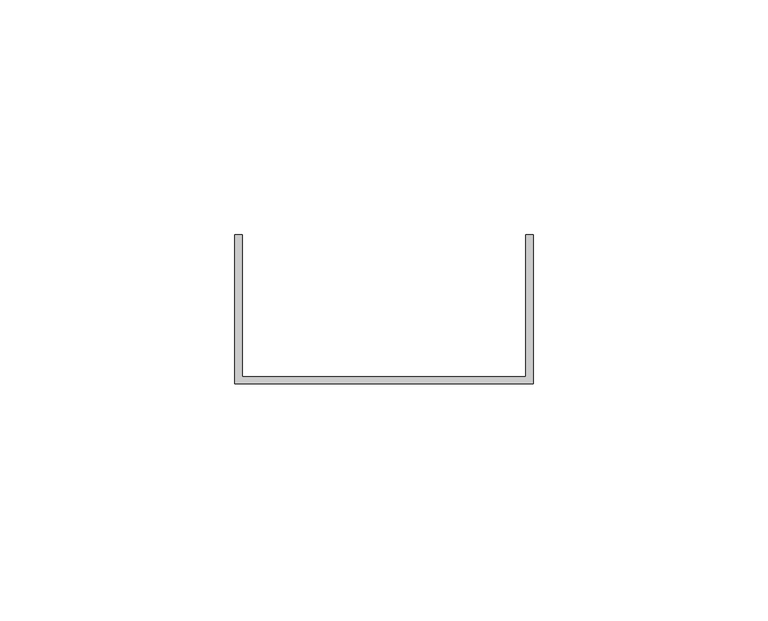
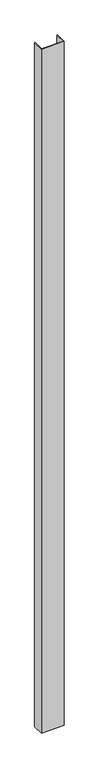
"""IFC4 building model written with IfcOpenShell, lengths in millimetres: proxy geometry, Generic Models 7:Generic Models 1:3:Generic Models 1:3 : Generic Models 7:Generic Models 1:305549:3:Generic Models 1:3:Generic Models 1:3 : Generic Models 7:Generic Models 1:305549:3 : Generic Models 7:Generic Models 1:3:Generic Models 1:3 : Generic Models 7:Generic Models 1:305549:301244:29 : Generic Models 7:Generic Models 1:3:Generic Models 1:3 : Generic Models 7:Generic Models 1:305549:3:Generic Models 1:3:Generic Models 1:3 : Generic Models 7:Generic Models 1:305549:3 : Generic Models 7:Generic Models 1:3:Generic Models 1:3 : Generic Models 7:Generic Models 1:305549:301244:308848."""

import ifcopenshell
import ifcopenshell.guid

model = None  # the IFC model being written
_history = None  # IfcOwnerHistory: only IFC2X3 demands one
_inside = {}  # id of a spatial element -> (the spatial element, [elements in it])
_under = {}  # id of a project, library or spatial element -> (it, [spatial elements below it])
_declared = {}  # id of a project -> (the project, [libraries it declares])
_typed = {}  # id of a type object -> (the type object, [elements of that type])
_made_of = {}  # id of a material, layer set ... -> (it, [elements and type objects made of it])


def new_model(schema):
    """Start an empty IFC model of exactly this schema.

    Asked for "IFC4X3", IfcOpenShell would pick the latest addendum, in which some entities
    have other attributes; the version numbers below select the first issue.
    IFC2X3 requires an IfcOwnerHistory on every rooted entity: one is made here for all.
    """
    global model, _history
    if schema == "IFC4X3":
        model = ifcopenshell.file(schema_version=(4, 3, 0, 0))
    else:
        model = ifcopenshell.file(schema=schema)
    _inside.clear()
    _under.clear()
    _declared.clear()
    _typed.clear()
    _made_of.clear()
    _history = None
    if model.schema == "IFC2X3":
        org = make("IfcOrganization", Name="unknown")
        user = make(
            "IfcPersonAndOrganization",
            ThePerson=make("IfcPerson", FamilyName="unknown"),
            TheOrganization=org,
        )
        app = make(
            "IfcApplication",
            ApplicationDeveloper=org,
            Version="unknown",
            ApplicationFullName="unknown",
            ApplicationIdentifier="unknown",
        )
        _history = make(
            "IfcOwnerHistory",
            OwningUser=user,
            OwningApplication=app,
            ChangeAction="ADDED",
            CreationDate=0,
        )
    return model


def make(cls, **values):
    """One entity of the class cls with the attributes given. An attribute that is None is left unset."""
    return model.create_entity(
        cls, **{name: value for name, value in values.items() if value is not None}
    )


def rooted(cls, **values):
    """An entity with a GlobalId (a new one), such as an element, a storey or a relation."""
    return make(cls, GlobalId=ifcopenshell.guid.new(), OwnerHistory=_history, **values)


def si_unit(unit_type, name, prefix=None):
    """IfcSIUnit, for example si_unit("LENGTHUNIT", "METRE", prefix="MILLI")."""
    return make("IfcSIUnit", UnitType=unit_type, Prefix=prefix, Name=name)


def assignment(units):
    """IfcUnitAssignment: the units of a project."""
    return None if units is None else make("IfcUnitAssignment", Units=units)


def point(xyz):
    """IfcCartesianPoint."""
    return None if xyz is None else make("IfcCartesianPoint", Coordinates=xyz)


def direction(xyz):
    """IfcDirection."""
    return None if xyz is None else make("IfcDirection", DirectionRatios=xyz)


def frame(location, z_axis=None, x_axis=None):
    """IfcAxis2Placement3D, a coordinate frame: its origin and axes. An axis left out is left unset."""
    return make(
        "IfcAxis2Placement3D",
        Location=point(location),
        Axis=direction(z_axis),
        RefDirection=direction(x_axis),
    )


def origin():
    """The frame at (0, 0, 0) with its axes left unset."""
    return frame((0.0, 0.0, 0.0))


def place(relative_to, where):
    """IfcLocalPlacement: puts the frame where relative to a parent placement (None: the world)."""
    return make(
        "IfcLocalPlacement", PlacementRelTo=relative_to, RelativePlacement=where
    )


def context(
    kind, dimensions, precision=None, world=None, true_north=None, identifier=None
):
    """IfcGeometricRepresentationContext, for example the 3D "Model" context."""
    return make(
        "IfcGeometricRepresentationContext",
        ContextIdentifier=identifier,
        ContextType=kind,
        CoordinateSpaceDimension=dimensions,
        Precision=precision,
        WorldCoordinateSystem=world,
        TrueNorth=true_north,
    )


def project(units=None, contexts=None):
    """IfcProject with its units and contexts."""
    return rooted(
        "IfcProject",
        Name="project",
        RepresentationContexts=contexts,
        UnitsInContext=assignment(units),
    )


def spatial(cls, under=None, at=None, **own):
    """A site, building, storey or space (cls), placed at a placement, below another one or the project."""
    s = rooted(cls, ObjectPlacement=at, **own)
    if under is not None:
        _under.setdefault(under.id(), (under, []))[1].append(s)
    return s


def polyline(points):
    """IfcPolyline through the points."""
    return make("IfcPolyline", Points=[point(p) for p in points])


def outline(outer, holes=None, kind="AREA"):
    """IfcArbitraryClosedProfileDef: a profile drawn as a closed curve; with holes, ...WithVoids."""
    if holes is None:
        return make("IfcArbitraryClosedProfileDef", ProfileType=kind, OuterCurve=outer)
    return make(
        "IfcArbitraryProfileDefWithVoids",
        ProfileType=kind,
        OuterCurve=outer,
        InnerCurves=holes,
    )


def extrude(swept, where, along, depth):
    """IfcExtrudedAreaSolid: the profile swept, set in the frame where, extruded along a direction by depth."""
    return make(
        "IfcExtrudedAreaSolid",
        SweptArea=swept,
        Position=where,
        ExtrudedDirection=direction(along),
        Depth=depth,
    )


def shape(context_of_items, identifier, shape_type, items):
    """IfcShapeRepresentation: the items that make up one representation, for example the "Body"."""
    return make(
        "IfcShapeRepresentation",
        ContextOfItems=context_of_items,
        RepresentationIdentifier=identifier,
        RepresentationType=shape_type,
        Items=items,
    )


def source(mapping_origin, context_of_items, identifier, shape_type, items):
    """IfcRepresentationMap: a shape defined once, which mapped items show again and again."""
    return make(
        "IfcRepresentationMap",
        MappingOrigin=mapping_origin,
        MappedRepresentation=shape(context_of_items, identifier, shape_type, items),
    )


def transform(
    local_origin,
    x_axis=None,
    y_axis=None,
    z_axis=None,
    scale=None,
    scale2=None,
    scale3=None,
    uniform=True,
):
    """IfcCartesianTransformationOperator3D, or its non-uniform kind. x_axis, y_axis, z_axis: its Axis1, 2, 3."""
    if uniform:
        return make(
            "IfcCartesianTransformationOperator3D",
            Axis1=direction(x_axis),
            Axis2=direction(y_axis),
            LocalOrigin=point(local_origin),
            Scale=scale,
            Axis3=direction(z_axis),
        )
    return make(
        "IfcCartesianTransformationOperator3DnonUniform",
        Axis1=direction(x_axis),
        Axis2=direction(y_axis),
        LocalOrigin=point(local_origin),
        Scale=scale,
        Axis3=direction(z_axis),
        Scale2=scale2,
        Scale3=scale3,
    )


def mapped(mapping_source, mapping_target):
    """IfcMappedItem: shows the shape of a source again, moved by a transform."""
    return make(
        "IfcMappedItem", MappingSource=mapping_source, MappingTarget=mapping_target
    )


def made_of(thing, what):
    """Note that an element or type object is made of a material, layer set ...; save() writes the relation."""
    if what is not None:
        _made_of.setdefault(what.id(), (what, []))[1].append(thing)
    return thing


def element(
    cls,
    number,
    at=None,
    inside=None,
    cuts=None,
    type_object=None,
    material=None,
    context=None,
    identifier="Body",
    shape_type=None,
    held_by="IfcProductDefinitionShape",
    body=None,
    shapes=None,
    **own,
):
    """One element of the class cls, such as IfcWall. Its Tag is "e" and its number.

    at: its placement. inside: the storey or other place that contains it. cuts: it is an
    opening in that element (IfcRelVoidsElement). A single representation is given by context,
    identifier, shape_type and body (its items); several are given by shapes. held_by: the class
    of the entity that holds the representations. save() writes the other relations.
    """
    e = rooted(cls, Tag="e%d" % number, ObjectPlacement=at, **own)
    if body is not None:
        shapes = [shape(context, identifier, shape_type, body)]
    if shapes is not None:
        e.Representation = make(held_by, Representations=shapes)
    if inside is not None:
        _inside.setdefault(inside.id(), (inside, []))[1].append(e)
    if cuts is not None:
        rooted(
            "IfcRelVoidsElement", RelatingBuildingElement=cuts, RelatedOpeningElement=e
        )
    if type_object is not None:
        _typed.setdefault(type_object.id(), (type_object, []))[1].append(e)
    return made_of(e, material)


def aggregate(whole, parts):
    """IfcRelAggregates: a whole, such as a stair, and the parts it consists of."""
    return rooted("IfcRelAggregates", RelatingObject=whole, RelatedObjects=parts)


def save(model, path):
    """Write the relations noted so far, then the file.

    IfcRelAggregates (storeys below a building ...), IfcRelContainedInSpatialStructure (elements
    in a storey), IfcRelDefinesByType, IfcRelAssociatesMaterial and IfcRelDeclares: one each for
    every whole, place, type object, material and project.
    """
    for whole, parts in _under.values():
        aggregate(whole, parts)
    for where, things in _inside.values():
        rooted(
            "IfcRelContainedInSpatialStructure",
            RelatedElements=things,
            RelatingStructure=where,
        )
    for kind, things in _typed.values():
        rooted("IfcRelDefinesByType", RelatedObjects=things, RelatingType=kind)
    for what, things in _made_of.values():
        rooted("IfcRelAssociatesMaterial", RelatedObjects=things, RelatingMaterial=what)
    for by, libraries in _declared.values():
        rooted("IfcRelDeclares", RelatingContext=by, RelatedDefinitions=libraries)
    model.write(path)


def generic_models_4e9104a0(model_context):
    return source(origin(), model_context, "Body", "SweptSolid", [
        extrude(outline(polyline([(579320.411724, -578666.2203133), (579320.411724, -578634.4703133), (579321.999224, -578634.4703133), (579321.999224, -578664.6328133), (579382.3242239, -578664.6328133), (579382.3242239, -578634.4703133), (579383.9117239, -578634.4703133), (579383.9117239, -578666.2203133), (579320.411724, -578666.2203133)])), frame((0.0, 0.0, 4133.81326), z_axis=(0.0, 0.0, 1.0), x_axis=(1.0, 0.0, 0.0)), (0.0, 0.0, 1.0), 2000.28674),
    ])


if __name__ == "__main__":
    model = new_model("IFC4")
    model_context = context("Model", 3, world=origin())
    ifc_project = project(units=[si_unit("LENGTHUNIT", "METRE", prefix="MILLI")], contexts=[model_context])
    site = spatial("IfcSite", under=ifc_project)
    building = spatial("IfcBuilding", under=site)
    placement = place(None, origin())
    generic_models_shape = generic_models_4e9104a0(model_context)
    element("IfcBuildingElementProxy", 1, Name="Generic Models 7:Generic Models 1:3:Generic Models 1:3 : Generic Models 7:Generic Models 1:305549:3:Generic Models 1:3:Generic Models 1:3 : Generic Models 7:Generic Models 1:305549:3 : Generic Models 7:Generic Models 1:3:Generic Models 1:3 : Generic Models 7:Generic Models 1:305549:301244:29 : Generic Models 7:Generic Models 1:3:Generic Models 1:3 : Generic Models 7:Generic Models 1:305549:3:Generic Models 1:3:Generic Models 1:3 : Generic Models 7:Generic Models 1:305549:3 : Generic Models 7:Generic Models 1:3:Generic Models 1:3 : Generic Models 7:Generic Models 1:305549:301244:308848", ObjectType="Generic Models 7:Generic Models 1:3:Generic Models 1:3 : Generic Models 7:Generic Models 1:305549:3:Generic Models 1:3:Generic Models 1:3 : Generic Models 7:Generic Models 1:305549:3 : Generic Models 7:Generic Models 1:3:Generic Models 1:3 : Generic Models 7:Generic Models 1:305549:301244:29 : Generic Models 7:Generic Models 1:3:Generic Models 1:3 : Generic Models 7:Generic Models 1:305549:3:Generic Models 1:3:Generic Models 1:3 : Generic Models 7:Generic Models 1:305549:3 : Generic Models 7:Generic Models 1:3:Generic Models 1:3 : Generic Models 7:Generic Models 1:305549:301244:308848", at=placement, inside=building, context=model_context, shape_type="MappedRepresentation", body=[
        mapped(generic_models_shape, transform((0.0, 0.0, 0.0), x_axis=(1.0, 0.0, 0.0), y_axis=(0.0, 1.0, 0.0), z_axis=(0.0, 0.0, 1.0))),
    ])
    save(model, "model.ifc")

# Revit data of these elements
# Type "Generic Models 7:Generic Models 1:3:Generic Models 1:3 : Generic Models 7:Generic Models 1:305549:3:Generic Models 1:3:Generic Models 1:3 : Generic Models 7:Generic Models 1:305549:3 : Generic Models 7:Generic Models 1:3:Generic Models 1:3 : Generic Models 7:Generic Models 1:305549:301244:29 : Generic Models 7:Generic Models 1:3:Generic Models 1:3 : Generic Models 7:Generic Models 1:305549:3:Generic Models 1:3:Generic Models 1:3 : Generic Models 7:Generic Models 1:305549:3 : Generic Models 7:Generic Models 1:3:Generic Models 1:3 : Generic Models 7:Generic Models 1:305549:301244:308848"
#   NameOverride = "Generic Models 7:Generic Models 1:3:Generic Models 1:3 : Generic Models 7:Generic Models 1:305549:3:Generic Models 1:3:Generic Models 1:3 : Generic Models 7:Generic Models 1:305549:3 : Generic Models 7:Generic Models 1:3:Generic Models 1:3 : Generic Models 7:Generic Models 1:305549:301244:308848"
#   ObjectTypeOverride = "Generic Models 1:3:Generic Models 1:3 : Generic Models 7:Generic Models 1:305549:3 : Generic Models 7:Generic Models 1:3:Generic Models 1:3 : Generic Models 7:Generic Models 1:305549:301244"
#   Reference = "Generic Models 1"
#   Tag = "308848"
# Element 1 (IfcBuildingElementProxy, "Generic Models 7:Generic Models 1:3:Generic Models 1:3 : Generic Models 7:Generic Models 1:305549:3:Generic Models 1:3:Generic Models 1:3 : Generic Models 7:Generic Models 1:305549:3 : Generic Models 7:Generic Models 1:3:Generic Models 1:3 : Generic Models 7:Generic Models 1:305549:301244:29 : Generic Models 7:Generic Models 1:3:Generic Models 1:3 : Generic Models 7:Generic Models 1:305549:3:Generic Models 1:3:Generic Models 1:3 : Generic Models 7:Generic Models 1:305549:3 : Generic Models 7:Generic Models 1:3:Generic Models 1:3 : Generic Models 7:Generic Models 1:305549:301244:308848")
#   Materials on its faces: "GALVANIZED U-CHANNEL (250T125-33)"
# Materials
#   "GALVANIZED U-CHANNEL (250T125-33)": class "Unassigned", colour RGB 202 201 200, transparency 0, Keynote = "M05451300.02", Cost = 0
